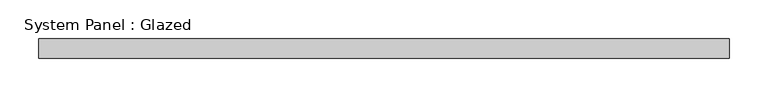
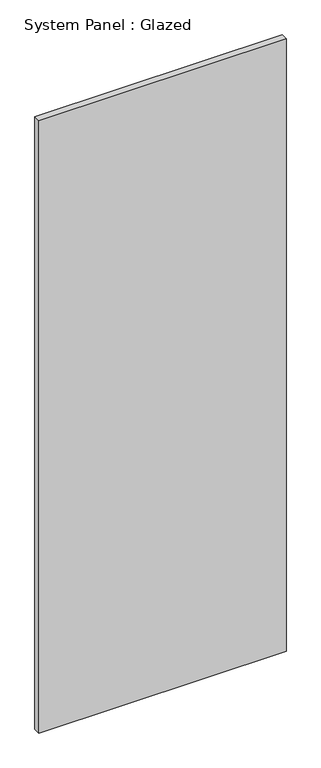
"""IFC4 building model written with IfcOpenShell, lengths in millimetres: plate geometry, System Panel : Glazed."""

from ifc_helpers import new_model, si_unit, origin, origin_with_axes, place, context, project, spatial, polyline, outline, extrude, source, transform, mapped, element, save


def system_panel_glazed_25e8ab93(model_context):
    return source(origin(), model_context, "Body", "SweptSolid", [
        extrude(outline(polyline([(443.75, 24.5), (-443.75, 24.5), (-443.75, 49.5), (443.75, 49.5), (443.75, 24.5)])), origin_with_axes(), (0.0, 0.0, 1.0), 2325.0),
    ])


if __name__ == "__main__":
    model = new_model("IFC4")
    model_context = context("Model", 3, world=origin())
    ifc_project = project(units=[si_unit("LENGTHUNIT", "METRE", prefix="MILLI")], contexts=[model_context])
    site = spatial("IfcSite", under=ifc_project)
    building = spatial("IfcBuilding", under=site)
    placement = place(None, origin())
    system_panel_glazed_shape = system_panel_glazed_25e8ab93(model_context)
    element("IfcPlate", 1, ObjectType="System Panel : Glazed", at=placement, inside=building, context=model_context, shape_type="MappedRepresentation", body=[
        mapped(system_panel_glazed_shape, transform((0.0, 0.0, 0.0), x_axis=(1.0, 0.0, 0.0), y_axis=(0.0, 1.0, 0.0), z_axis=(0.0, 0.0, 1.0))),
    ])
    save(model, "model.ifc")

# Revit data of these elements
# Type "System Panel : Glazed"
#   Construction Type Id = "GSP4R"
#   Analytic Construction = "1/8 in Pilkington single glazing"
#   Visual Light Transmittance = 0.9
#   Solar Heat Gain Coefficient = 0.86
#   Heat Transfer Coefficient (U) = 6.7069 W/(m²·K)
#   Define Thermal Properties by = 1
# Element 1 (IfcPlate, "System Panel : Glazed")
#   Materials on its faces: "Glass"
# Materials
#   "Glass": class "Glass", colour RGB 0 128 192, transparency 0.9, Description = "Soda Lime Glass", Cost = 0
